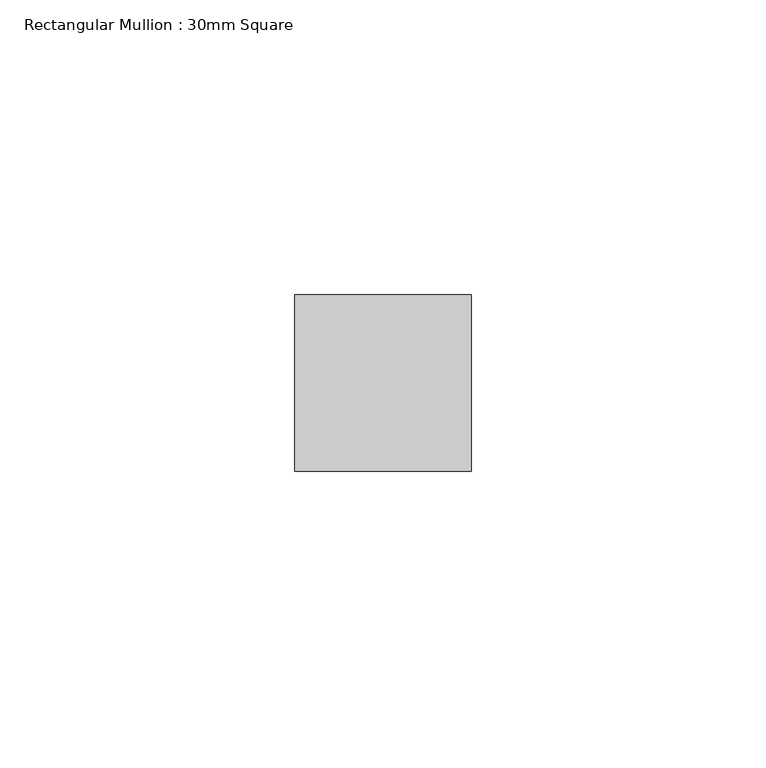
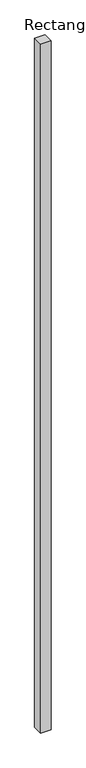
"""IFC4 building model written with IfcOpenShell, lengths in millimetres: member geometry, Rectangular Mullion : 30mm Square."""

from ifc_helpers import new_model, si_unit, frame, origin, place, context, project, spatial, polyline, outline, extrude, source, transform, mapped, element, save


def rectangular_mullion_30mm_square_ef009769(model_context):
    return source(origin(), model_context, "Body", "SweptSolid", [
        extrude(outline(polyline([(15.0, 15.0), (15.0, -15.0), (-15.0, -15.0), (-15.0, 15.0), (15.0, 15.0)])), frame((0.0, 0.0, -2098.4348088), z_axis=(0.0, 0.0, 1.0), x_axis=(1.0, 0.0, 0.0)), (0.0, 0.0, 1.0), 2098.4348088),
    ])


if __name__ == "__main__":
    model = new_model("IFC4")
    model_context = context("Model", 3, world=origin())
    ifc_project = project(units=[si_unit("LENGTHUNIT", "METRE", prefix="MILLI")], contexts=[model_context])
    site = spatial("IfcSite", under=ifc_project)
    building = spatial("IfcBuilding", under=site)
    placement = place(None, origin())
    rectangular_mullion_30mm_square_shape = rectangular_mullion_30mm_square_ef009769(model_context)
    element("IfcMember", 1, ObjectType="Rectangular Mullion : 30mm Square", at=placement, inside=building, context=model_context, shape_type="MappedRepresentation", body=[
        mapped(rectangular_mullion_30mm_square_shape, transform((0.0, 0.0, 0.0), x_axis=(1.0, 0.0, 0.0), y_axis=(0.0, 1.0, 0.0), z_axis=(0.0, 0.0, 1.0))),
    ])
    save(model, "model.ifc")

# Revit data of these elements
# Type "Rectangular Mullion : 30mm Square"
#   built-in parameter 1007304 = 0.0984252 (stored number, unit not read)
#   built-in parameter 1007301 = 0.0492126 (stored number, unit not read)
#   built-in parameter 1007300 = 0.0492126 (stored number, unit not read)
# Element 1 (IfcMember, "Rectangular Mullion : 30mm Square")
#   Materials on its faces: "Aluminum"
# Materials
#   "Aluminum": class "Metal", colour RGB 244 244 244, transparency 0, Description = "Aluminum 6061", Cost = 0
